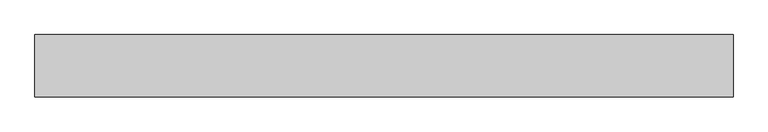
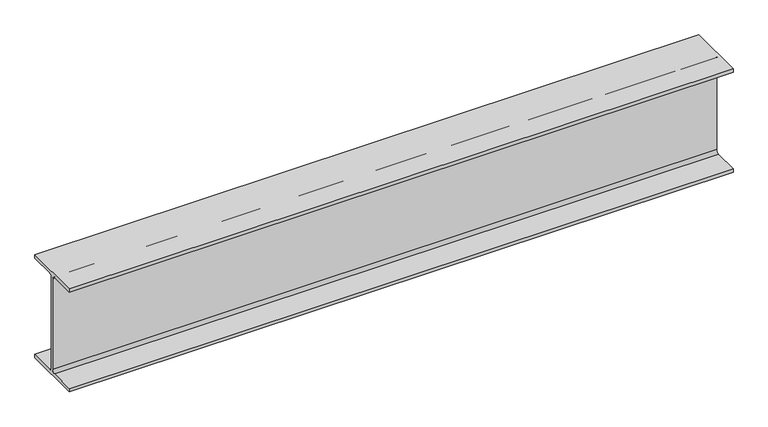
"""IFC4 building model written with IfcOpenShell, lengths in millimetres: beam geometry, Old_Steel Beam_H-KSD3502 : H_SB_ASB_H-194×150x6x9."""

from ifc_helpers import new_model, si_unit, point, frame, frame_2d, origin, place, context, project, spatial, polyline, circle_curve, trimmed, segment, composite_curve, outline, extrude, source, transform, mapped, element, save


def beam_802452f5(model_context):
    return source(origin(), model_context, "Body", "SweptSolid", [
        extrude(outline(composite_curve([segment(polyline([(82.5, -141.5), (82.5, -151.7), (-82.5, -151.7), (-82.5, -141.5), (-11.9, -141.5)]), True, "CONTINUOUS"), segment(trimmed(circle_curve(frame_2d((-11.9, -132.6)), 8.9), [point((-11.9, -141.5))], [point((-3.0, -132.6))], True, "CARTESIAN"), True, "CONTINUOUS"), segment(polyline([(-3.0, -132.6), (-3.0, 132.6)]), True, "CONTINUOUS"), segment(trimmed(circle_curve(frame_2d((-11.9, 132.6)), 8.9), [point((-3.0, 132.6))], [point((-11.9, 141.5))], True, "CARTESIAN"), True, "CONTINUOUS"), segment(polyline([(-11.9, 141.5), (-82.5, 141.5), (-82.5, 151.7), (82.5, 151.7), (82.5, 141.5), (11.9, 141.5)]), True, "CONTINUOUS"), segment(trimmed(circle_curve(frame_2d((11.9, 132.6)), 8.9), [point((11.9, 141.5))], [point((3.0, 132.6))], True, "CARTESIAN"), True, "CONTINUOUS"), segment(polyline([(3.0, 132.6), (3.0, -132.6)]), True, "CONTINUOUS"), segment(trimmed(circle_curve(frame_2d((11.9, -132.6)), 8.9), [point((3.0, -132.6))], [point((11.9, -141.5))], True, "CARTESIAN"), True, "CONTINUOUS"), segment(polyline([(11.9, -141.5), (82.5, -141.5)]), True, "CONTINUOUS")], self_intersect=False)), frame((-853.4240734, 0.0, 0.0), z_axis=(1.0, 0.0, 0.0), x_axis=(0.0, 1.0, 0.0)), (0.0, 0.0, 1.0), 1846.5746098),
    ])


if __name__ == "__main__":
    model = new_model("IFC4")
    model_context = context("Model", 3, world=origin())
    ifc_project = project(units=[si_unit("LENGTHUNIT", "METRE", prefix="MILLI")], contexts=[model_context])
    site = spatial("IfcSite", under=ifc_project)
    building = spatial("IfcBuilding", under=site)
    placement = place(None, origin())
    beam_shape = beam_802452f5(model_context)
    element("IfcBeam", 1, ObjectType="Old_Steel Beam_H-KSD3502 : H_SB_ASB_H-194×150x6x9", at=placement, inside=building, context=model_context, shape_type="MappedRepresentation", body=[
        mapped(beam_shape, transform((0.0, 0.0, 0.0), x_axis=(1.0, 0.0, 0.0), y_axis=(0.0, 1.0, 0.0), z_axis=(0.0, 0.0, 1.0))),
    ])
    save(model, "model.ifc")

# Revit data of these elements
# Type "Old_Steel Beam_H-KSD3502 : H_SB_ASB_H-194×150x6x9"
#   Width = 15.0 cm
#   Web Thickness = 0.6 cm
#   Web Fillet = 1.3 cm
#   Warping Constant = 43316.0 cm⁶
#   Torsional Moment of Inertia = 8.622 cm⁴
#   Torsional Modulus = 1.0 cm³
#   Section Area = 39.01 cm²
#   Plastic Modulus weak axis = 104.0 cm³
#   Plastic Modulus strong axis = 309.0 cm³
#   Perimeter = 0.95 m²/m
#   Nominal Weight = 30.60 kgf/m
#   Moment of Inertia weak axis = 507.00 cm⁴
#   Moment of Inertia strong axis = 2690.00 cm⁴
#   Height = 19.4 cm
#   Flange Thickness = 0.9 cm
#   Elastic Modulus weak axis = 67.6 cm³
#   Elastic Modulus strong axis = 277.0 cm³
#   Centroid Vertical = 9.7 cm
#   Centroid Horizontal = 7.5 cm
#   Length [instance default] = 1.5240 m
#   Structural Material [instance default] = Steel, 45-345
#   Assembly Code = ""
# Element 1 (IfcBeam, "Old_Steel Beam_H-KSD3502 : H_SB_ASB_H-194×150x6x9")
#   Structural Material = none
# Materials
#   "Steel, 45-345": class "Metal", colour RGB 189 187 185, transparency 0, Description = "Steel 345 MPa", Cost = 0
